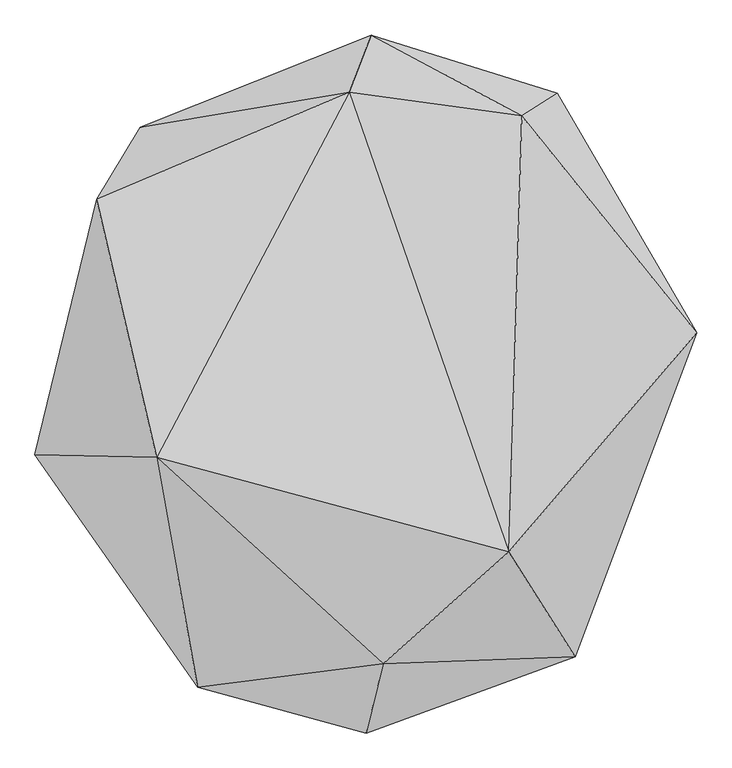
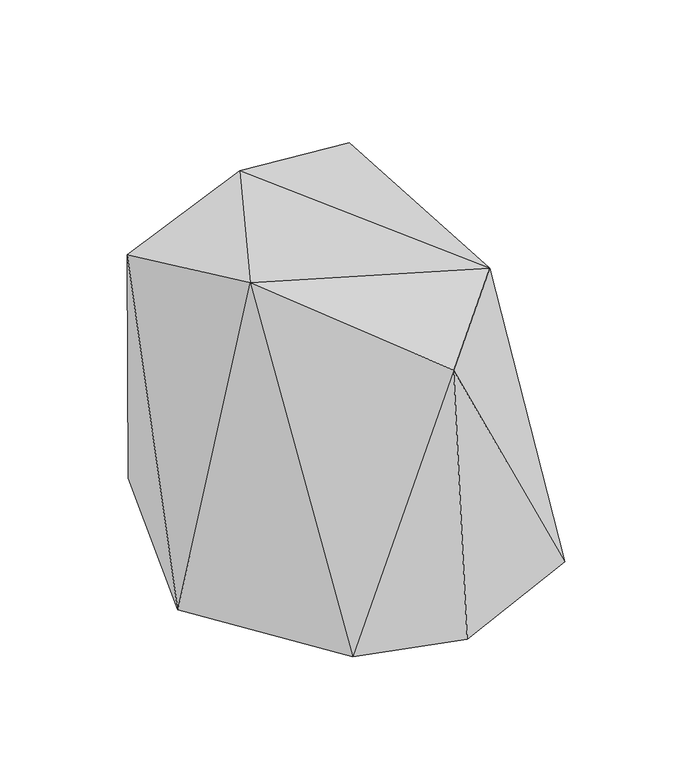
"""IFC4 building model written with IfcOpenShell, lengths in millimetres: geographic element geometry, Enscape AssetDefinition - Bush 124 Pampas Grass : Enscape AssetDefinition - Bush 124 Pampas Grass."""

import ifcopenshell
import ifcopenshell.guid

model = None  # the IFC model being written
_history = None  # IfcOwnerHistory: only IFC2X3 demands one
_inside = {}  # id of a spatial element -> (the spatial element, [elements in it])
_under = {}  # id of a project, library or spatial element -> (it, [spatial elements below it])
_declared = {}  # id of a project -> (the project, [libraries it declares])
_typed = {}  # id of a type object -> (the type object, [elements of that type])
_made_of = {}  # id of a material, layer set ... -> (it, [elements and type objects made of it])


def new_model(schema):
    """Start an empty IFC model of exactly this schema.

    Asked for "IFC4X3", IfcOpenShell would pick the latest addendum, in which some entities
    have other attributes; the version numbers below select the first issue.
    IFC2X3 requires an IfcOwnerHistory on every rooted entity: one is made here for all.
    """
    global model, _history
    if schema == "IFC4X3":
        model = ifcopenshell.file(schema_version=(4, 3, 0, 0))
    else:
        model = ifcopenshell.file(schema=schema)
    _inside.clear()
    _under.clear()
    _declared.clear()
    _typed.clear()
    _made_of.clear()
    _history = None
    if model.schema == "IFC2X3":
        org = make("IfcOrganization", Name="unknown")
        user = make(
            "IfcPersonAndOrganization",
            ThePerson=make("IfcPerson", FamilyName="unknown"),
            TheOrganization=org,
        )
        app = make(
            "IfcApplication",
            ApplicationDeveloper=org,
            Version="unknown",
            ApplicationFullName="unknown",
            ApplicationIdentifier="unknown",
        )
        _history = make(
            "IfcOwnerHistory",
            OwningUser=user,
            OwningApplication=app,
            ChangeAction="ADDED",
            CreationDate=0,
        )
    return model


def make(cls, **values):
    """One entity of the class cls with the attributes given. An attribute that is None is left unset."""
    return model.create_entity(
        cls, **{name: value for name, value in values.items() if value is not None}
    )


def rooted(cls, **values):
    """An entity with a GlobalId (a new one), such as an element, a storey or a relation."""
    return make(cls, GlobalId=ifcopenshell.guid.new(), OwnerHistory=_history, **values)


def si_unit(unit_type, name, prefix=None):
    """IfcSIUnit, for example si_unit("LENGTHUNIT", "METRE", prefix="MILLI")."""
    return make("IfcSIUnit", UnitType=unit_type, Prefix=prefix, Name=name)


def assignment(units):
    """IfcUnitAssignment: the units of a project."""
    return None if units is None else make("IfcUnitAssignment", Units=units)


def point(xyz):
    """IfcCartesianPoint."""
    return None if xyz is None else make("IfcCartesianPoint", Coordinates=xyz)


def direction(xyz):
    """IfcDirection."""
    return None if xyz is None else make("IfcDirection", DirectionRatios=xyz)


def frame(location, z_axis=None, x_axis=None):
    """IfcAxis2Placement3D, a coordinate frame: its origin and axes. An axis left out is left unset."""
    return make(
        "IfcAxis2Placement3D",
        Location=point(location),
        Axis=direction(z_axis),
        RefDirection=direction(x_axis),
    )


def origin():
    """The frame at (0, 0, 0) with its axes left unset."""
    return frame((0.0, 0.0, 0.0))


def place(relative_to, where):
    """IfcLocalPlacement: puts the frame where relative to a parent placement (None: the world)."""
    return make(
        "IfcLocalPlacement", PlacementRelTo=relative_to, RelativePlacement=where
    )


def context(
    kind, dimensions, precision=None, world=None, true_north=None, identifier=None
):
    """IfcGeometricRepresentationContext, for example the 3D "Model" context."""
    return make(
        "IfcGeometricRepresentationContext",
        ContextIdentifier=identifier,
        ContextType=kind,
        CoordinateSpaceDimension=dimensions,
        Precision=precision,
        WorldCoordinateSystem=world,
        TrueNorth=true_north,
    )


def project(units=None, contexts=None):
    """IfcProject with its units and contexts."""
    return rooted(
        "IfcProject",
        Name="project",
        RepresentationContexts=contexts,
        UnitsInContext=assignment(units),
    )


def spatial(cls, under=None, at=None, **own):
    """A site, building, storey or space (cls), placed at a placement, below another one or the project."""
    s = rooted(cls, ObjectPlacement=at, **own)
    if under is not None:
        _under.setdefault(under.id(), (under, []))[1].append(s)
    return s


def faces_of(points, faces, orient=None, outer=None):
    """IfcFace entities. A face is a list of loops; a loop is a list of indices into points, from 0.

    orient and outer hold one flag for each loop. By default every Orientation is true, the
    first loop of a face is its IfcFaceOuterBound and the others are IfcFaceBound.
    """
    made = []
    for i, loops in enumerate(faces):
        bounds = []
        for j, loop in enumerate(loops):
            is_outer = j == 0 if outer is None else outer[i][j]
            bounds.append(
                make(
                    "IfcFaceOuterBound" if is_outer else "IfcFaceBound",
                    Bound=make("IfcPolyLoop", Polygon=[points[k] for k in loop]),
                    Orientation=True if orient is None else orient[i][j],
                )
            )
        made.append(make("IfcFace", Bounds=bounds))
    return made


def faceted_brep(points, faces, orient=None, outer=None, voids=None):
    """IfcFacetedBrep: a solid bounded by flat faces; with voids (closed shells), ...WithVoids."""
    shared = [point(p) for p in points]
    hull = make("IfcClosedShell", CfsFaces=faces_of(shared, faces, orient, outer))
    if voids is None:
        return make("IfcFacetedBrep", Outer=hull)
    return make(
        "IfcFacetedBrepWithVoids",
        Outer=hull,
        Voids=[
            make(cls, CfsFaces=faces_of(shared, fs, o, b)) for cls, fs, o, b in voids
        ],
    )


def shape(context_of_items, identifier, shape_type, items):
    """IfcShapeRepresentation: the items that make up one representation, for example the "Body"."""
    return make(
        "IfcShapeRepresentation",
        ContextOfItems=context_of_items,
        RepresentationIdentifier=identifier,
        RepresentationType=shape_type,
        Items=items,
    )


def source(mapping_origin, context_of_items, identifier, shape_type, items):
    """IfcRepresentationMap: a shape defined once, which mapped items show again and again."""
    return make(
        "IfcRepresentationMap",
        MappingOrigin=mapping_origin,
        MappedRepresentation=shape(context_of_items, identifier, shape_type, items),
    )


def transform(
    local_origin,
    x_axis=None,
    y_axis=None,
    z_axis=None,
    scale=None,
    scale2=None,
    scale3=None,
    uniform=True,
):
    """IfcCartesianTransformationOperator3D, or its non-uniform kind. x_axis, y_axis, z_axis: its Axis1, 2, 3."""
    if uniform:
        return make(
            "IfcCartesianTransformationOperator3D",
            Axis1=direction(x_axis),
            Axis2=direction(y_axis),
            LocalOrigin=point(local_origin),
            Scale=scale,
            Axis3=direction(z_axis),
        )
    return make(
        "IfcCartesianTransformationOperator3DnonUniform",
        Axis1=direction(x_axis),
        Axis2=direction(y_axis),
        LocalOrigin=point(local_origin),
        Scale=scale,
        Axis3=direction(z_axis),
        Scale2=scale2,
        Scale3=scale3,
    )


def mapped(mapping_source, mapping_target):
    """IfcMappedItem: shows the shape of a source again, moved by a transform."""
    return make(
        "IfcMappedItem", MappingSource=mapping_source, MappingTarget=mapping_target
    )


def made_of(thing, what):
    """Note that an element or type object is made of a material, layer set ...; save() writes the relation."""
    if what is not None:
        _made_of.setdefault(what.id(), (what, []))[1].append(thing)
    return thing


def element(
    cls,
    number,
    at=None,
    inside=None,
    cuts=None,
    type_object=None,
    material=None,
    context=None,
    identifier="Body",
    shape_type=None,
    held_by="IfcProductDefinitionShape",
    body=None,
    shapes=None,
    **own,
):
    """One element of the class cls, such as IfcWall. Its Tag is "e" and its number.

    at: its placement. inside: the storey or other place that contains it. cuts: it is an
    opening in that element (IfcRelVoidsElement). A single representation is given by context,
    identifier, shape_type and body (its items); several are given by shapes. held_by: the class
    of the entity that holds the representations. save() writes the other relations.
    """
    e = rooted(cls, Tag="e%d" % number, ObjectPlacement=at, **own)
    if body is not None:
        shapes = [shape(context, identifier, shape_type, body)]
    if shapes is not None:
        e.Representation = make(held_by, Representations=shapes)
    if inside is not None:
        _inside.setdefault(inside.id(), (inside, []))[1].append(e)
    if cuts is not None:
        rooted(
            "IfcRelVoidsElement", RelatingBuildingElement=cuts, RelatedOpeningElement=e
        )
    if type_object is not None:
        _typed.setdefault(type_object.id(), (type_object, []))[1].append(e)
    return made_of(e, material)


def aggregate(whole, parts):
    """IfcRelAggregates: a whole, such as a stair, and the parts it consists of."""
    return rooted("IfcRelAggregates", RelatingObject=whole, RelatedObjects=parts)


def save(model, path):
    """Write the relations noted so far, then the file.

    IfcRelAggregates (storeys below a building ...), IfcRelContainedInSpatialStructure (elements
    in a storey), IfcRelDefinesByType, IfcRelAssociatesMaterial and IfcRelDeclares: one each for
    every whole, place, type object, material and project.
    """
    for whole, parts in _under.values():
        aggregate(whole, parts)
    for where, things in _inside.values():
        rooted(
            "IfcRelContainedInSpatialStructure",
            RelatedElements=things,
            RelatingStructure=where,
        )
    for kind, things in _typed.values():
        rooted("IfcRelDefinesByType", RelatedObjects=things, RelatingType=kind)
    for what, things in _made_of.values():
        rooted("IfcRelAssociatesMaterial", RelatedObjects=things, RelatingMaterial=what)
    for by, libraries in _declared.values():
        rooted("IfcRelDeclares", RelatingContext=by, RelatedDefinitions=libraries)
    model.write(path)


def geographic_element_9c8827ca(model_context):
    return source(origin(), model_context, "Body", "Brep", [
        faceted_brep([(-264.2639875, -536.5539789, 88.6489972), (-339.3009901, -117.5350025, 1082.6699734), (-560.995996, -112.7799973, 88.6489972), (11.8039995, 547.9059815, 923.6680269), (-448.6410022, 352.7109921, 928.7919998), (73.4319985, -493.712008, 881.5860152), (302.7119935, -289.655, 1010.3069544), (-369.4530129, 484.5449924, 88.6489972), (-107.4849963, -0.627, -7.4829999), (42.5710008, -619.6249723, 88.6449963), (423.4899879, -480.5459976, 124.5009974), (644.8199749, 109.6689999, 125.455007), (326.1559904, 504.7410131, 931.0209751), (52.0480014, 652.4310112, 88.6489972), (391.2200034, 546.1400151, 88.6489972)], [[[0, 1, 2]], [[3, 4, 1]], [[4, 2, 1]], [[0, 5, 1]], [[6, 3, 1]], [[5, 6, 1]], [[2, 7, 8]], [[2, 8, 0]], [[7, 2, 4]], [[0, 9, 5]], [[0, 8, 9]], [[10, 5, 9]], [[10, 6, 5]], [[11, 12, 6]], [[12, 3, 6]], [[10, 11, 6]], [[9, 8, 10]], [[10, 8, 11]], [[13, 14, 8]], [[8, 7, 13]], [[8, 14, 11]], [[13, 7, 3]], [[3, 7, 4]], [[14, 13, 12]], [[12, 13, 3]], [[11, 14, 12]]]),
    ])


if __name__ == "__main__":
    model = new_model("IFC4")
    model_context = context("Model", 3, world=origin())
    ifc_project = project(units=[si_unit("LENGTHUNIT", "METRE", prefix="MILLI")], contexts=[model_context])
    site = spatial("IfcSite", under=ifc_project)
    building = spatial("IfcBuilding", under=site)
    placement = place(None, origin())
    geographic_element_shape = geographic_element_9c8827ca(model_context)
    element("IfcGeographicElement", 1, ObjectType="Enscape AssetDefinition - Bush 124 Pampas Grass : Enscape AssetDefinition - Bush 124 Pampas Grass", at=placement, inside=building, context=model_context, shape_type="MappedRepresentation", body=[
        mapped(geographic_element_shape, transform((0.0, 0.0, 0.0), x_axis=(1.0, 0.0, 0.0), y_axis=(0.0, 1.0, 0.0), z_axis=(0.0, 0.0, 1.0))),
    ])
    save(model, "model.ifc")

# Revit data of these elements
# Type "Enscape AssetDefinition - Bush 124 Pampas Grass : Enscape AssetDefinition - Bush 124 Pampas Grass"
#   EnscapeAssetSource = "REMOTE"
#   EnscapeAssetId = "c051ca4c-e4a4-4b28-9467-8725a50cb4a2"
#   Height = 1.08267 m
#   EnscapeNativeAssetHeight = 1.08267 m
#   Default Elevation = 0
